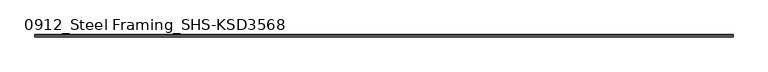
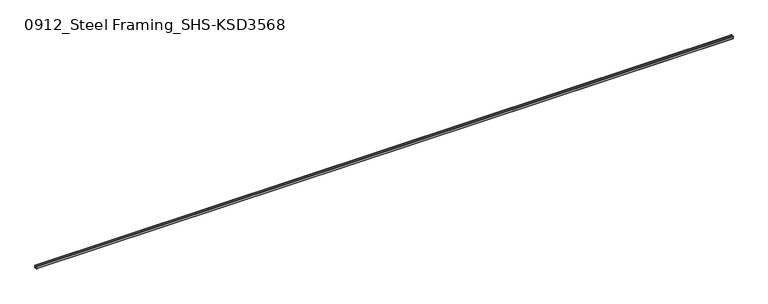
"""IFC4 building model written with IfcOpenShell, lengths in millimetres: beam geometry, 0912_Steel Framing_SHS-KSD3568 : H_SB_ASB_SHS-150x150x6."""

import ifcopenshell
import ifcopenshell.guid

model = None  # the IFC model being written
_history = None  # IfcOwnerHistory: only IFC2X3 demands one
_inside = {}  # id of a spatial element -> (the spatial element, [elements in it])
_under = {}  # id of a project, library or spatial element -> (it, [spatial elements below it])
_declared = {}  # id of a project -> (the project, [libraries it declares])
_typed = {}  # id of a type object -> (the type object, [elements of that type])
_made_of = {}  # id of a material, layer set ... -> (it, [elements and type objects made of it])


def new_model(schema):
    """Start an empty IFC model of exactly this schema.

    Asked for "IFC4X3", IfcOpenShell would pick the latest addendum, in which some entities
    have other attributes; the version numbers below select the first issue.
    IFC2X3 requires an IfcOwnerHistory on every rooted entity: one is made here for all.
    """
    global model, _history
    if schema == "IFC4X3":
        model = ifcopenshell.file(schema_version=(4, 3, 0, 0))
    else:
        model = ifcopenshell.file(schema=schema)
    _inside.clear()
    _under.clear()
    _declared.clear()
    _typed.clear()
    _made_of.clear()
    _history = None
    if model.schema == "IFC2X3":
        org = make("IfcOrganization", Name="unknown")
        user = make(
            "IfcPersonAndOrganization",
            ThePerson=make("IfcPerson", FamilyName="unknown"),
            TheOrganization=org,
        )
        app = make(
            "IfcApplication",
            ApplicationDeveloper=org,
            Version="unknown",
            ApplicationFullName="unknown",
            ApplicationIdentifier="unknown",
        )
        _history = make(
            "IfcOwnerHistory",
            OwningUser=user,
            OwningApplication=app,
            ChangeAction="ADDED",
            CreationDate=0,
        )
    return model


def make(cls, **values):
    """One entity of the class cls with the attributes given. An attribute that is None is left unset."""
    return model.create_entity(
        cls, **{name: value for name, value in values.items() if value is not None}
    )


def rooted(cls, **values):
    """An entity with a GlobalId (a new one), such as an element, a storey or a relation."""
    return make(cls, GlobalId=ifcopenshell.guid.new(), OwnerHistory=_history, **values)


def si_unit(unit_type, name, prefix=None):
    """IfcSIUnit, for example si_unit("LENGTHUNIT", "METRE", prefix="MILLI")."""
    return make("IfcSIUnit", UnitType=unit_type, Prefix=prefix, Name=name)


def assignment(units):
    """IfcUnitAssignment: the units of a project."""
    return None if units is None else make("IfcUnitAssignment", Units=units)


def point(xyz):
    """IfcCartesianPoint."""
    return None if xyz is None else make("IfcCartesianPoint", Coordinates=xyz)


def direction(xyz):
    """IfcDirection."""
    return None if xyz is None else make("IfcDirection", DirectionRatios=xyz)


def frame(location, z_axis=None, x_axis=None):
    """IfcAxis2Placement3D, a coordinate frame: its origin and axes. An axis left out is left unset."""
    return make(
        "IfcAxis2Placement3D",
        Location=point(location),
        Axis=direction(z_axis),
        RefDirection=direction(x_axis),
    )


def frame_2d(location, x_axis=None):
    """IfcAxis2Placement2D, a coordinate frame in the plane: its origin and x axis."""
    return make(
        "IfcAxis2Placement2D", Location=point(location), RefDirection=direction(x_axis)
    )


def origin():
    """The frame at (0, 0, 0) with its axes left unset."""
    return frame((0.0, 0.0, 0.0))


def place(relative_to, where):
    """IfcLocalPlacement: puts the frame where relative to a parent placement (None: the world)."""
    return make(
        "IfcLocalPlacement", PlacementRelTo=relative_to, RelativePlacement=where
    )


def context(
    kind, dimensions, precision=None, world=None, true_north=None, identifier=None
):
    """IfcGeometricRepresentationContext, for example the 3D "Model" context."""
    return make(
        "IfcGeometricRepresentationContext",
        ContextIdentifier=identifier,
        ContextType=kind,
        CoordinateSpaceDimension=dimensions,
        Precision=precision,
        WorldCoordinateSystem=world,
        TrueNorth=true_north,
    )


def project(units=None, contexts=None):
    """IfcProject with its units and contexts."""
    return rooted(
        "IfcProject",
        Name="project",
        RepresentationContexts=contexts,
        UnitsInContext=assignment(units),
    )


def spatial(cls, under=None, at=None, **own):
    """A site, building, storey or space (cls), placed at a placement, below another one or the project."""
    s = rooted(cls, ObjectPlacement=at, **own)
    if under is not None:
        _under.setdefault(under.id(), (under, []))[1].append(s)
    return s


def polyline(points):
    """IfcPolyline through the points."""
    return make("IfcPolyline", Points=[point(p) for p in points])


def circle_curve(where, radius):
    """IfcCircle in the frame where."""
    return make("IfcCircle", Position=where, Radius=radius)


def trimmed(basis, trim1, trim2, sense, master):
    """IfcTrimmedCurve: the piece of a basis curve between two trims."""
    return make(
        "IfcTrimmedCurve",
        BasisCurve=basis,
        Trim1=trim1,
        Trim2=trim2,
        SenseAgreement=sense,
        MasterRepresentation=master,
    )


def segment(curve, same_sense, transition):
    """IfcCompositeCurveSegment."""
    return make(
        "IfcCompositeCurveSegment",
        Transition=transition,
        SameSense=same_sense,
        ParentCurve=curve,
    )


def composite_curve(segments, self_intersect=None):
    """IfcCompositeCurve: segments joined end to end."""
    return make("IfcCompositeCurve", Segments=segments, SelfIntersect=self_intersect)


def outline(outer, holes=None, kind="AREA"):
    """IfcArbitraryClosedProfileDef: a profile drawn as a closed curve; with holes, ...WithVoids."""
    if holes is None:
        return make("IfcArbitraryClosedProfileDef", ProfileType=kind, OuterCurve=outer)
    return make(
        "IfcArbitraryProfileDefWithVoids",
        ProfileType=kind,
        OuterCurve=outer,
        InnerCurves=holes,
    )


def extrude(swept, where, along, depth):
    """IfcExtrudedAreaSolid: the profile swept, set in the frame where, extruded along a direction by depth."""
    return make(
        "IfcExtrudedAreaSolid",
        SweptArea=swept,
        Position=where,
        ExtrudedDirection=direction(along),
        Depth=depth,
    )


def shape(context_of_items, identifier, shape_type, items):
    """IfcShapeRepresentation: the items that make up one representation, for example the "Body"."""
    return make(
        "IfcShapeRepresentation",
        ContextOfItems=context_of_items,
        RepresentationIdentifier=identifier,
        RepresentationType=shape_type,
        Items=items,
    )


def source(mapping_origin, context_of_items, identifier, shape_type, items):
    """IfcRepresentationMap: a shape defined once, which mapped items show again and again."""
    return make(
        "IfcRepresentationMap",
        MappingOrigin=mapping_origin,
        MappedRepresentation=shape(context_of_items, identifier, shape_type, items),
    )


def transform(
    local_origin,
    x_axis=None,
    y_axis=None,
    z_axis=None,
    scale=None,
    scale2=None,
    scale3=None,
    uniform=True,
):
    """IfcCartesianTransformationOperator3D, or its non-uniform kind. x_axis, y_axis, z_axis: its Axis1, 2, 3."""
    if uniform:
        return make(
            "IfcCartesianTransformationOperator3D",
            Axis1=direction(x_axis),
            Axis2=direction(y_axis),
            LocalOrigin=point(local_origin),
            Scale=scale,
            Axis3=direction(z_axis),
        )
    return make(
        "IfcCartesianTransformationOperator3DnonUniform",
        Axis1=direction(x_axis),
        Axis2=direction(y_axis),
        LocalOrigin=point(local_origin),
        Scale=scale,
        Axis3=direction(z_axis),
        Scale2=scale2,
        Scale3=scale3,
    )


def mapped(mapping_source, mapping_target):
    """IfcMappedItem: shows the shape of a source again, moved by a transform."""
    return make(
        "IfcMappedItem", MappingSource=mapping_source, MappingTarget=mapping_target
    )


def made_of(thing, what):
    """Note that an element or type object is made of a material, layer set ...; save() writes the relation."""
    if what is not None:
        _made_of.setdefault(what.id(), (what, []))[1].append(thing)
    return thing


def element(
    cls,
    number,
    at=None,
    inside=None,
    cuts=None,
    type_object=None,
    material=None,
    context=None,
    identifier="Body",
    shape_type=None,
    held_by="IfcProductDefinitionShape",
    body=None,
    shapes=None,
    **own,
):
    """One element of the class cls, such as IfcWall. Its Tag is "e" and its number.

    at: its placement. inside: the storey or other place that contains it. cuts: it is an
    opening in that element (IfcRelVoidsElement). A single representation is given by context,
    identifier, shape_type and body (its items); several are given by shapes. held_by: the class
    of the entity that holds the representations. save() writes the other relations.
    """
    e = rooted(cls, Tag="e%d" % number, ObjectPlacement=at, **own)
    if body is not None:
        shapes = [shape(context, identifier, shape_type, body)]
    if shapes is not None:
        e.Representation = make(held_by, Representations=shapes)
    if inside is not None:
        _inside.setdefault(inside.id(), (inside, []))[1].append(e)
    if cuts is not None:
        rooted(
            "IfcRelVoidsElement", RelatingBuildingElement=cuts, RelatedOpeningElement=e
        )
    if type_object is not None:
        _typed.setdefault(type_object.id(), (type_object, []))[1].append(e)
    return made_of(e, material)


def aggregate(whole, parts):
    """IfcRelAggregates: a whole, such as a stair, and the parts it consists of."""
    return rooted("IfcRelAggregates", RelatingObject=whole, RelatedObjects=parts)


def save(model, path):
    """Write the relations noted so far, then the file.

    IfcRelAggregates (storeys below a building ...), IfcRelContainedInSpatialStructure (elements
    in a storey), IfcRelDefinesByType, IfcRelAssociatesMaterial and IfcRelDeclares: one each for
    every whole, place, type object, material and project.
    """
    for whole, parts in _under.values():
        aggregate(whole, parts)
    for where, things in _inside.values():
        rooted(
            "IfcRelContainedInSpatialStructure",
            RelatedElements=things,
            RelatingStructure=where,
        )
    for kind, things in _typed.values():
        rooted("IfcRelDefinesByType", RelatedObjects=things, RelatingType=kind)
    for what, things in _made_of.values():
        rooted("IfcRelAssociatesMaterial", RelatedObjects=things, RelatingMaterial=what)
    for by, libraries in _declared.values():
        rooted("IfcRelDeclares", RelatingContext=by, RelatedDefinitions=libraries)
    model.write(path)


def beam_0912_steel_framing_shs_ksd3568_b3aa3b39(model_context):
    return source(origin(), model_context, "Body", "SweptSolid", [
        extrude(outline(composite_curve([segment(trimmed(circle_curve(frame_2d((-63.0, 63.0)), 12.0), [point((-75.0, 63.0))], [point((-63.0, 75.0))], False, "CARTESIAN"), True, "CONTINUOUS"), segment(polyline([(-63.0, 75.0), (63.0, 75.0)]), True, "CONTINUOUS"), segment(trimmed(circle_curve(frame_2d((63.0, 63.0)), 12.0), [point((63.0, 75.0))], [point((75.0, 63.0))], False, "CARTESIAN"), True, "CONTINUOUS"), segment(polyline([(75.0, 63.0), (75.0, -63.0)]), True, "CONTINUOUS"), segment(trimmed(circle_curve(frame_2d((63.0, -63.0)), 12.0), [point((75.0, -63.0))], [point((63.0, -75.0))], False, "CARTESIAN"), True, "CONTINUOUS"), segment(polyline([(63.0, -75.0), (-63.0, -75.0)]), True, "CONTINUOUS"), segment(trimmed(circle_curve(frame_2d((-63.0, -63.0)), 12.0), [point((-63.0, -75.0))], [point((-75.0, -63.0))], False, "CARTESIAN"), True, "CONTINUOUS"), segment(polyline([(-75.0, -63.0), (-75.0, 63.0)]), True, "CONTINUOUS")], self_intersect=False), holes=[composite_curve([segment(polyline([(63.0, 69.0), (-63.0, 69.0)]), True, "CONTINUOUS"), segment(trimmed(circle_curve(frame_2d((-63.0, 63.0)), 6.0), [point((-63.0, 69.0))], [point((-69.0, 63.0))], True, "CARTESIAN"), True, "CONTINUOUS"), segment(polyline([(-69.0, 63.0), (-69.0, -63.0)]), True, "CONTINUOUS"), segment(trimmed(circle_curve(frame_2d((-63.0, -63.0)), 6.0), [point((-69.0, -63.0))], [point((-63.0, -69.0))], True, "CARTESIAN"), True, "CONTINUOUS"), segment(polyline([(-63.0, -69.0), (63.0, -69.0)]), True, "CONTINUOUS"), segment(trimmed(circle_curve(frame_2d((63.0, -63.0)), 6.0), [point((63.0, -69.0))], [point((69.0, -63.0))], True, "CARTESIAN"), True, "CONTINUOUS"), segment(polyline([(69.0, -63.0), (69.0, 63.0)]), True, "CONTINUOUS"), segment(trimmed(circle_curve(frame_2d((63.0, 63.0)), 6.0), [point((69.0, 63.0))], [point((63.0, 69.0))], True, "CARTESIAN"), True, "CONTINUOUS")], self_intersect=False)]), frame((-20440.0, 0.0, 0.0), z_axis=(1.0, 0.0, 0.0), x_axis=(0.0, 1.0, 0.0)), (0.0, 0.0, 1.0), 40880.0),
    ])


if __name__ == "__main__":
    model = new_model("IFC4")
    model_context = context("Model", 3, world=origin())
    ifc_project = project(units=[si_unit("LENGTHUNIT", "METRE", prefix="MILLI")], contexts=[model_context])
    site = spatial("IfcSite", under=ifc_project)
    building = spatial("IfcBuilding", under=site)
    placement = place(None, origin())
    beam_0912_steel_framing_shs_ksd3568_shape = beam_0912_steel_framing_shs_ksd3568_b3aa3b39(model_context)
    element("IfcBeam", 1, ObjectType="0912_Steel Framing_SHS-KSD3568 : H_SB_ASB_SHS-150x150x6", at=placement, inside=building, context=model_context, shape_type="MappedRepresentation", body=[
        mapped(beam_0912_steel_framing_shs_ksd3568_shape, transform((0.0, 0.0, 0.0), x_axis=(1.0, 0.0, 0.0), y_axis=(0.0, 1.0, 0.0), z_axis=(0.0, 0.0, 1.0))),
    ])
    save(model, "model.ifc")

# Revit data of these elements
# Type "0912_Steel Framing_SHS-KSD3568 : H_SB_ASB_SHS-150x150x6"
#   H_WM Code_1 = "S01AA002-00001 | Main Steel Structure Fabrication Work | Shelter/Building | Medium Steel - Standard (90KG/M>Weight≥30KG/M) | Material: (   )"
#   H_WM Code_2 = "S03AA028-00001 | Main Steel Structure Erection Work | Shelter/Building | Medium Steel (90KG/M>Weight≥30KG/M) | Material: (   )"
#   H_WM Code_3 = "S01AA010-00001 | Main Steel Structure Fabrication Work | Shelter/Building | Steel Painting/Coating | for Non-Fireproofed Steel Surface, Surface Preparation, Primer, Second & Final Coat | Material: (   )"
#   H_Q'ty Cal Type Tag = "SB-Q2"
#   Perimeter = 0.60 m²/m
#   Nominal Weight = 26.40 kgf/m
#   Length [instance default] = 1.0000 m
#   b = 0.1500 m
#   h = 0.1500 m
#   tr = 0.0120 m
#   t = 0.0060 m
#   A = 28.36 m²
#   Structural Material [instance default] = Steel, 45-345
# Element 1 (IfcBeam, "0912_Steel Framing_SHS-KSD3568 : H_SB_ASB_SHS-150x150x6")
#   Structural Material = none
# Materials
#   "Steel, 45-345": class "Metal", colour RGB 189 187 185, transparency 0, Description = "Steel 345 MPa", Cost = 0
